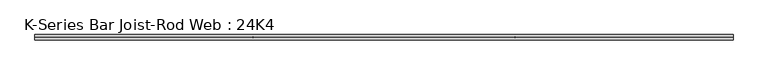
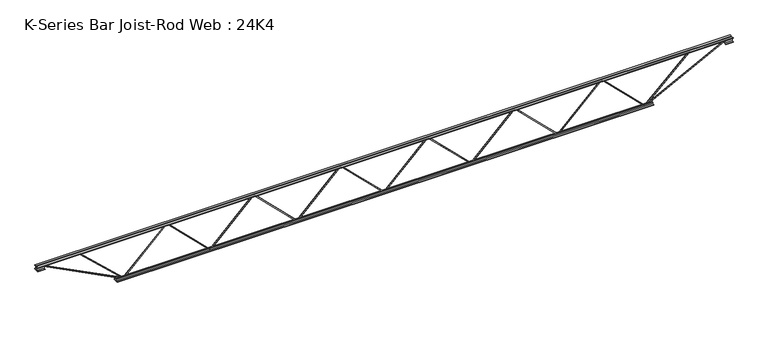
"""IFC4 building model written with IfcOpenShell, lengths in millimetres: beam geometry, K-Series Bar Joist-Rod Web : 24K4."""

from ifc_helpers import new_model, si_unit, frame, origin, place, context, project, spatial, polyline, outline, extrude, source, transform, mapped, element, save


def k_series_bar_joist_rod_web_24k4_0bbdf4ea(model_context):
    return source(origin(), model_context, "Body", "SweptSolid", [
        extrude(outline(polyline([(-293.6875, 1223.16875), (-303.2125, 1223.16875), (-303.2125, 1228.2971284), (293.6875, 1833.5315034), (293.6875, 1835.9747466), (-303.2125, 2441.2091216), (-303.2125, 2446.3375), (-293.6875, 2446.3375), (-293.6875, 2445.1158784), (303.2125, 1839.8815034), (303.2125, 1829.6247466), (-293.6875, 1224.3903716), (-293.6875, 1223.16875)])), frame((0.0, -4.7625, 0.0), z_axis=(0.0, 1.0, 0.0), x_axis=(0.0, 0.0, 1.0)), (0.0, 0.0, 1.0), 9.525),
        extrude(outline(polyline([(-293.6875, 0.0), (-303.2125, 0.0), (-303.2125, 5.1283784), (293.6875, 610.3627534), (293.6875, 612.8059966), (-303.2125, 1218.0403716), (-303.2125, 1223.16875), (-293.6875, 1223.16875), (-293.6875, 1221.9471284), (303.2125, 616.7127534), (303.2125, 606.4559966), (-293.6875, 1.2216216), (-293.6875, 0.0)])), frame((0.0, -4.7625, 0.0), z_axis=(0.0, 1.0, 0.0), x_axis=(0.0, 0.0, 1.0)), (0.0, 0.0, 1.0), 9.525),
        extrude(outline(polyline([(-293.6875, -1223.16875), (-303.2125, -1223.16875), (-303.2125, -1218.0403716), (293.6875, -612.8059966), (293.6875, -610.3627534), (-303.2125, -5.1283784), (-303.2125, 0.0), (-293.6875, 0.0), (-293.6875, -1.2216216), (303.2125, -606.4559966), (303.2125, -616.7127534), (-293.6875, -1221.9471284), (-293.6875, -1223.16875)])), frame((0.0, -4.7625, 0.0), z_axis=(0.0, 1.0, 0.0), x_axis=(0.0, 0.0, 1.0)), (0.0, 0.0, 1.0), 9.525),
        extrude(outline(polyline([(-293.6875, -2446.3375), (-303.2125, -2446.3375), (-303.2125, -2441.2091216), (293.6875, -1835.9747466), (293.6875, -1833.5315034), (-303.2125, -1228.2971284), (-303.2125, -1223.16875), (-293.6875, -1223.16875), (-293.6875, -1224.3903716), (303.2125, -1829.6247466), (303.2125, -1839.8815034), (-293.6875, -2445.1158784), (-293.6875, -2446.3375)])), frame((0.0, -4.7625, 0.0), z_axis=(0.0, 1.0, 0.0), x_axis=(0.0, 0.0, 1.0)), (0.0, 0.0, 1.0), 9.525),
        extrude(outline(polyline([(-293.6875, 2446.3375), (-303.2125, 2446.3375), (-303.2125, 2451.4658784), (293.6875, 3056.7002534), (293.6875, 3059.1434966), (-303.2125, 3664.3778716), (-303.2125, 3669.50625), (-293.6875, 3669.50625), (-293.6875, 3668.2846284), (303.2125, 3063.0502534), (303.2125, 3052.7934966), (-293.6875, 2447.5591216), (-293.6875, 2446.3375)])), frame((0.0, -4.7625, 0.0), z_axis=(0.0, 1.0, 0.0), x_axis=(0.0, 0.0, 1.0)), (0.0, 0.0, 1.0), 9.525),
        extrude(outline(polyline([(-293.6875, -3669.50625), (-303.2125, -3669.50625), (-303.2125, -3664.3778716), (293.6875, -3059.1434966), (293.6875, -3056.7002534), (-303.2125, -2451.4658784), (-303.2125, -2446.3375), (-293.6875, -2446.3375), (-293.6875, -2447.5591216), (303.2125, -3052.7934966), (303.2125, -3063.0502534), (-293.6875, -3668.2846284), (-293.6875, -3669.50625)])), frame((0.0, -4.7625, 0.0), z_axis=(0.0, 1.0, 0.0), x_axis=(0.0, 0.0, 1.0)), (0.0, 0.0, 1.0), 9.525),
        extrude(outline(polyline([(4.7625, 304.8), (36.5125, 304.8), (36.5125, 298.45), (11.1125, 298.45), (11.1125, 273.05), (4.7625, 273.05), (4.7625, 304.8)])), frame((-4888.70625, 0.0, 0.0), z_axis=(1.0, 0.0, 0.0), x_axis=(0.0, 1.0, 0.0)), (0.0, 0.0, 1.0), 9777.4125),
        extrude(outline(polyline([(-4.7625, 304.8), (-4.7625, 273.05), (-11.1125, 273.05), (-11.1125, 298.45), (-36.5125, 298.45), (-36.5125, 304.8), (-4.7625, 304.8)])), frame((-4888.70625, 0.0, 0.0), z_axis=(1.0, 0.0, 0.0), x_axis=(0.0, 1.0, 0.0)), (0.0, 0.0, 1.0), 9777.4125),
        extrude(outline(polyline([(-4.7625, 241.3), (-36.5125, 241.3), (-36.5125, 247.65), (-11.1125, 247.65), (-11.1125, 273.05), (-4.7625, 273.05), (-4.7625, 241.3)])), frame((-4888.70625, 0.0, 0.0), z_axis=(1.0, 0.0, 0.0), x_axis=(0.0, 1.0, 0.0)), (0.0, 0.0, 1.0), 101.6),
        extrude(outline(polyline([(36.5125, 241.3), (4.7625, 241.3), (4.7625, 273.05), (11.1125, 273.05), (11.1125, 247.65), (36.5125, 247.65), (36.5125, 241.3)])), frame((-4888.70625, 0.0, 0.0), z_axis=(1.0, 0.0, 0.0), x_axis=(0.0, 1.0, 0.0)), (0.0, 0.0, 1.0), 101.6),
        extrude(outline(polyline([(4.7625, 241.3), (4.7625, 273.05), (11.1125, 273.05), (11.1125, 247.65), (36.5125, 247.65), (36.5125, 241.3), (4.7625, 241.3)])), frame((4787.10625, 0.0, 0.0), z_axis=(1.0, 0.0, 0.0), x_axis=(0.0, 1.0, 0.0)), (0.0, 0.0, 1.0), 101.6),
        extrude(outline(polyline([(-4.7625, 241.3), (-36.5125, 241.3), (-36.5125, 247.65), (-11.1125, 247.65), (-11.1125, 273.05), (-4.7625, 273.05), (-4.7625, 241.3)])), frame((4787.10625, 0.0, 0.0), z_axis=(1.0, 0.0, 0.0), x_axis=(0.0, 1.0, 0.0)), (0.0, 0.0, 1.0), 101.6),
        extrude(outline(polyline([(4.7625, -304.8), (4.7625, -273.05), (11.1125, -273.05), (11.1125, -298.45), (36.5125, -298.45), (36.5125, -304.8), (4.7625, -304.8)])), frame((-3771.10625, 0.0, 0.0), z_axis=(1.0, 0.0, 0.0), x_axis=(0.0, 1.0, 0.0)), (0.0, 0.0, 1.0), 7542.2125),
        extrude(outline(polyline([(-4.7625, -304.8), (-36.5125, -304.8), (-36.5125, -298.45), (-11.1125, -298.45), (-11.1125, -273.05), (-4.7625, -273.05), (-4.7625, -304.8)])), frame((-3771.10625, 0.0, 0.0), z_axis=(1.0, 0.0, 0.0), x_axis=(0.0, 1.0, 0.0)), (0.0, 0.0, 1.0), 7542.2125),
        extrude(outline(polyline([(0.0, -9.525), (0.0, 0.0), (1255.2457966, 0.0), (1255.2457966, -9.525), (0.0, -9.525)])), frame((-4789.2745654, 4.7625, 268.8097388), z_axis=(0.4552893158665215, 0.0, 0.8903435510283628), x_axis=(0.8903435510283628, 0.0, -0.4552893158665215)), (0.0, 0.0, 1.0), 9.525),
        extrude(outline(polyline([(0.0, -9.525), (0.0, 0.0), (837.0470105, 0.0), (837.0470105, -9.525), (0.0, -9.525)])), frame((-4284.3422569, 4.7625, 269.5703023), z_axis=(0.6827573515565595, 0.0, 0.7306451935758372), x_axis=(0.7306451935758372, 0.0, -0.6827573515565595)), (0.0, 0.0, 1.0), 9.525),
        extrude(outline(polyline([(0.0, -9.525), (0.0, 0.0), (1255.2457966, 0.0), (1255.2457966, -9.525), (0.0, -9.525)])), frame((4789.2745654, -4.7625, 268.8097388), z_axis=(-0.4552893158665133, 0.0, 0.890343551028367), x_axis=(-0.890343551028367, 0.0, -0.4552893158665133)), (0.0, 0.0, 1.0), 9.525),
        extrude(outline(polyline([(0.0, -9.525), (0.0, 0.0), (837.0470105, 0.0), (837.0470105, -9.525), (0.0, -9.525)])), frame((4284.3422569, -4.7625, 269.5703023), z_axis=(-0.6827573515565561, 0.0, 0.7306451935758403), x_axis=(-0.7306451935758403, 0.0, -0.6827573515565561)), (0.0, 0.0, 1.0), 9.525),
    ])


if __name__ == "__main__":
    model = new_model("IFC4")
    model_context = context("Model", 3, world=origin())
    ifc_project = project(units=[si_unit("LENGTHUNIT", "METRE", prefix="MILLI")], contexts=[model_context])
    site = spatial("IfcSite", under=ifc_project)
    building = spatial("IfcBuilding", under=site)
    placement = place(None, origin())
    k_series_bar_joist_rod_web_24k4_shape = k_series_bar_joist_rod_web_24k4_0bbdf4ea(model_context)
    element("IfcBeam", 1, ObjectType="K-Series Bar Joist-Rod Web : 24K4", at=placement, inside=building, context=model_context, shape_type="MappedRepresentation", body=[
        mapped(k_series_bar_joist_rod_web_24k4_shape, transform((0.0, 0.0, 0.0), x_axis=(1.0, 0.0, 0.0), y_axis=(0.0, 1.0, 0.0), z_axis=(0.0, 0.0, 1.0))),
    ])
    save(model, "model.ifc")

# Revit data of these elements
# Type "K-Series Bar Joist-Rod Web : 24K4"
#   Assembly Code = "B1010350"
#   Wt = 8.4
#   Web Thickness = 9.525 mm
#   Start Offset [instance default] = 0 mm
#   Start Extension [instance default] = 0 mm
#   Seat Length = 101.6 mm
#   Seat Depth = 63.5 mm
#   PanelArrayLength [instance default] = 4876.8 mm
#   Panel [instance default] = 1219.2 mm
#   End Offset [instance default] = 0 mm
#   End Extension [instance default] = 0 mm
#   End Panel = 1219.2 mm
#   Cord Leg = 31.75 mm
#   Chord Thickness = 6.35 mm
#   Length [instance default] = 7315.2 mm
#   Depth = 609.6 mm
#   PanelArrayNum [instance default] = 4
#   Structural Material = Steel ASTM A500, Grade C, Round
# Element 1 (IfcBeam, "K-Series Bar Joist-Rod Web : 24K4")
#   PanelArrayLength = 7339.013 mm
#   Panel = 1223.169 mm
#   PanelArrayNum = 6
#   Materials on its faces: "Steel ASTM A500, Grade C, Round"
# Materials
#   "Steel ASTM A500, Grade C, Round": class "Metal", colour RGB 202 101 0, transparency 0, Description = "Carbon steel", Cost = 0
